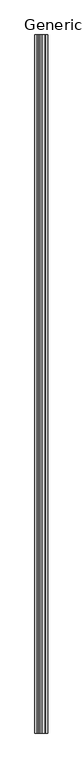
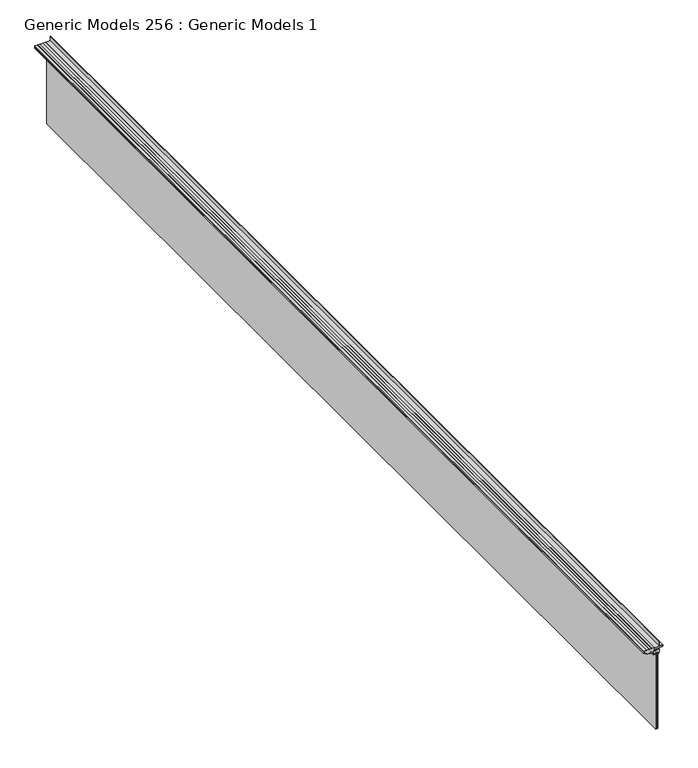
"""IFC4 building model written with IfcOpenShell, lengths in millimetres: proxy geometry, Generic Models 256 : Generic Models 1."""

from ifc_helpers import new_model, si_unit, point, frame, frame_2d, origin, place, context, project, spatial, polyline, circle_curve, trimmed, segment, composite_curve, outline, extrude, source, transform, mapped, element, save


def generic_models_256_generic_models_1_7edc17b0(model_context):
    return source(origin(), model_context, "Body", "SweptSolid", [
        extrude(outline(composite_curve([segment(polyline([(129190.1437953, 4830.4400913), (129182.1935781, 4830.4400913), (129182.1935781, 4838.3902843), (129180.2124005, 4838.3902843), (129180.2124005, 4830.4400913), (129170.2809815, 4830.4400913), (129170.2809815, 4840.7524463), (129169.468192, 4841.5398982), (129169.468192, 4844.7148982), (129165.5057885, 4844.7148982), (129165.5057885, 4846.3150913), (129162.3307885, 4850.2520602), (129162.3307885, 4851.8522533), (129159.943192, 4851.8522533), (129159.943192, 4870.9022533), (129153.6113595, 4870.9022533), (129153.6113595, 4900.3154773), (129156.7863595, 4900.3154773), (129156.7863595, 4897.2675044), (129165.4731595, 4897.2675044), (129165.4731595, 4879.7415044), (129167.7591595, 4879.7415044), (129167.7591595, 4897.2675044), (129168.698956, 4897.2675044), (129168.698956, 4905.6748401), (129176.649149, 4905.6748401), (129176.649149, 4907.6561145), (129170.2302095, 4907.6561145), (129170.2302095, 4911.6692416), (129175.1070021, 4911.6692416), (129175.1070021, 4946.6196416), (129177.529372, 4974.4834416), (129186.4607953, 4974.4834416), (129186.4607953, 4966.579876), (129188.7467953, 4966.579876), (129188.7467953, 4972.929876), (129190.1437953, 4972.929876), (129190.1437953, 4948.0420416), (129225.5108823, 4948.0420416)]), True, "CONTINUOUS"), segment(trimmed(circle_curve(frame_2d((129225.513342, 4947.3435419)), 0.6985041), [point((129225.5108823, 4948.0420416))], [point((129225.5156829, 4946.6450416))], False, "CARTESIAN"), True, "CONTINUOUS"), segment(polyline([(129225.5156829, 4946.6450416), (129190.1437953, 4946.6450416), (129190.1437953, 4910.1758738), (129186.9687953, 4910.1758738), (129186.9687953, 4907.8898738), (129190.1437953, 4907.8898738), (129190.1437953, 4890.7904913), (129188.0609953, 4890.7904913), (129188.0609953, 4887.6154913), (129190.1437953, 4887.6154913), (129190.1437953, 4870.5883916), (129186.9687953, 4870.5883916), (129186.9687953, 4868.3023877), (129190.1437953, 4868.3023877), (129190.1437953, 4850.7946386), (129186.9687953, 4850.7946386), (129186.9687953, 4848.5086347), (129190.1437953, 4848.5086347), (129190.1437953, 4830.4400913)]), True, "CONTINUOUS")], self_intersect=False)), frame((0.0, -1504.2676118, 0.0), z_axis=(0.0, 1.0, 0.0), x_axis=(0.0, 0.0, 1.0)), (0.0, 0.0, 1.0), 7886.7),
        extrude(outline(composite_curve([segment(polyline([(129141.2868845, 4938.1431837), (129137.0514453, 4938.1431837), (129137.0514453, 4939.2790416), (129135.0250715, 4939.2790416), (129135.2146218, 4941.7220811), (129143.0204453, 4944.2574416), (129143.0204453, 4946.6450416), (129165.3216453, 4946.6450416)]), True, "CONTINUOUS"), segment(trimmed(circle_curve(frame_2d((129165.3216453, 4944.2574416)), 2.3876), [point((129165.3216453, 4946.6450416))], [point((129167.7092453, 4944.2574416))], False, "CARTESIAN"), True, "CONTINUOUS"), segment(polyline([(129167.7092453, 4944.2574416), (129167.7092453, 4941.6920416), (129165.6772453, 4941.6920416), (129165.6772453, 4940.0156416), (129162.3752453, 4940.0156416), (129162.3752453, 4938.1106416), (129170.3000453, 4938.1106416), (129170.3000453, 4932.4972416), (129164.9914453, 4932.4972416), (129164.9914453, 4920.3052416)]), True, "CONTINUOUS"), segment(trimmed(circle_curve(frame_2d((129164.9914453, 4918.3240416)), 1.9812), [point((129164.9914453, 4920.3052416))], [point((129164.9914453, 4916.3428416))], True, "CARTESIAN"), True, "CONTINUOUS"), segment(polyline([(129164.9914453, 4916.3428416), (129164.9914453, 4903.0078416)]), True, "CONTINUOUS"), segment(trimmed(circle_curve(frame_2d((129164.1786453, 4903.0078416)), 0.8128), [point((129164.9914453, 4903.0078416))], [point((129164.1786453, 4902.1950416))], False, "CARTESIAN"), True, "CONTINUOUS"), segment(polyline([(129164.1786453, 4902.1950416), (129145.8906453, 4902.1950416), (129145.8906453, 4904.0755596), (129144.2897565, 4904.0755596), (129144.2897565, 4902.4753596), (129136.7459565, 4902.4753596), (129136.7459565, 4906.2432791), (129134.5836065, 4906.2432791), (129133.5709565, 4918.0709596), (129143.5023565, 4918.0709596), (129145.8906453, 4915.6826708), (129145.8906453, 4937.1200416), (129142.3100265, 4937.1200416), (129141.2868845, 4938.1431837)]), True, "CONTINUOUS")], self_intersect=False)), frame((0.0, -1504.2676118, 0.0), z_axis=(0.0, 1.0, 0.0), x_axis=(0.0, 0.0, 1.0)), (0.0, 0.0, 1.0), 7886.7),
        extrude(outline(polyline([(4923.6272096, -1504.2676118), (4918.8647096, -1504.2676118), (4918.8647096, 6382.4323882), (4923.6272096, 6382.4323882), (4923.6272096, -1504.2676118)])), frame((0.0, 0.0, 128542.7593472), z_axis=(0.0, 0.0, 1.0), x_axis=(1.0, 0.0, 0.0)), (0.0, 0.0, 1.0), 602.3375481),
        extrude(outline(polyline([(4930.7700416, -1504.2676118), (4924.4209596, -1504.2676118), (4924.4209596, 6382.4323882), (4930.7700416, 6382.4323882), (4930.7700416, -1504.2676118)])), frame((0.0, 0.0, 129138.7468953), z_axis=(0.0, 0.0, 1.0), x_axis=(1.0, 0.0, 0.0)), (0.0, 0.0, 1.0), 6.35),
        extrude(outline(polyline([(4936.3262916, -1504.2676118), (4931.5637916, -1504.2676118), (4931.5637916, 6382.4323882), (4936.3262916, 6382.4323882), (4936.3262916, -1504.2676118)])), frame((0.0, 0.0, 128542.7593472), z_axis=(0.0, 0.0, 1.0), x_axis=(1.0, 0.0, 0.0)), (0.0, 0.0, 1.0), 602.3375481),
    ])


if __name__ == "__main__":
    model = new_model("IFC4")
    model_context = context("Model", 3, world=origin())
    ifc_project = project(units=[si_unit("LENGTHUNIT", "METRE", prefix="MILLI")], contexts=[model_context])
    site = spatial("IfcSite", under=ifc_project)
    building = spatial("IfcBuilding", under=site)
    placement = place(None, origin())
    generic_models_256_generic_models_1_shape = generic_models_256_generic_models_1_7edc17b0(model_context)
    element("IfcBuildingElementProxy", 1, Name="Generic Models 256 : Generic Models 1", ObjectType="Generic Models 256 : Generic Models 1", at=placement, inside=building, context=model_context, shape_type="MappedRepresentation", body=[
        mapped(generic_models_256_generic_models_1_shape, transform((0.0, 0.0, 0.0), x_axis=(1.0, 0.0, 0.0), y_axis=(0.0, 1.0, 0.0), z_axis=(0.0, 0.0, 1.0))),
    ])
    save(model, "model.ifc")

# Revit data of these elements
# Element 1 (IfcBuildingElementProxy, "Generic Models 256 : Generic Models 1")
#   Materials on its faces: "_WINDOW PER SCHEDULE"
# Materials
#   "_WINDOW PER SCHEDULE": class "Generic", colour RGB 255 255 255, transparency 0, Cost = 0
